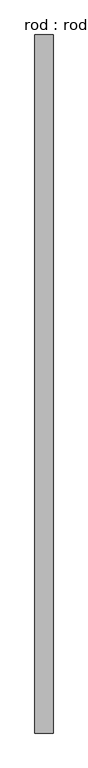
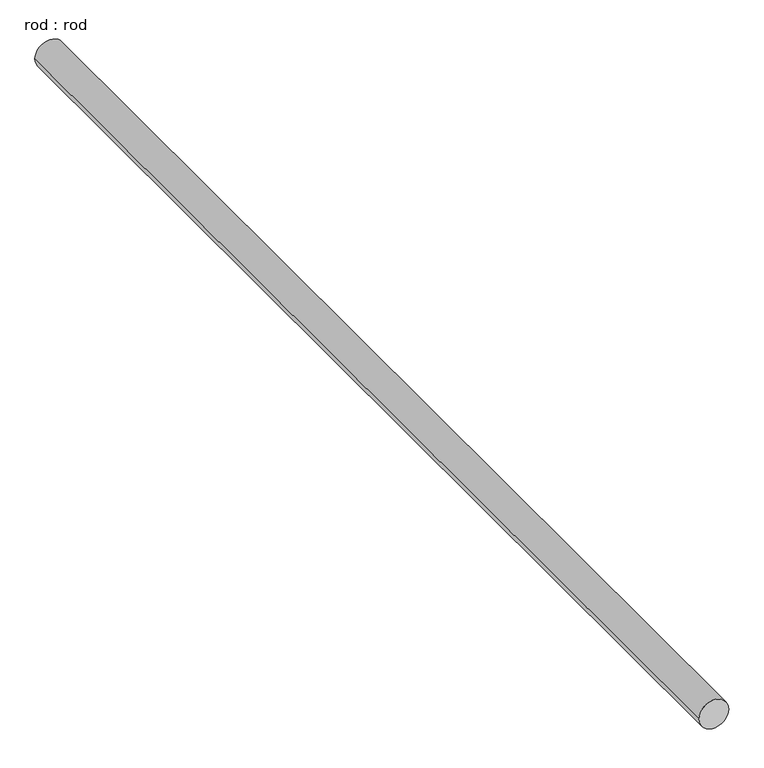
"""IFC4 building model written with IfcOpenShell, lengths in millimetres: proxy geometry, rod : rod."""

from ifc_helpers import new_model, si_unit, point, frame, frame_2d, origin, place, context, project, spatial, circle_curve, trimmed, segment, composite_curve, outline, extrude, source, transform, mapped, element, save


def rod_rod_69a24432(model_context):
    return source(origin(), model_context, "Body", "SweptSolid", [
        extrude(outline(composite_curve([segment(trimmed(circle_curve(frame_2d((0.0108462, 0.0)), 200.0), [point((0.0108462, 200.0))], [point((0.0108462, -200.0))], False, "CARTESIAN"), True, "CONTINUOUS"), segment(trimmed(circle_curve(frame_2d((0.0108462, 0.0)), 200.0), [point((0.0108462, -200.0))], [point((0.0108462, 200.0))], False, "CARTESIAN"), True, "CONTINUOUS")], self_intersect=False)), frame((0.0, -3607.5856259, 0.0), z_axis=(0.0, 1.0, 0.0), x_axis=(0.0, 0.0, 1.0)), (0.0, 0.0, 1.0), 15400.6284824),
    ])


if __name__ == "__main__":
    model = new_model("IFC4")
    model_context = context("Model", 3, world=origin())
    ifc_project = project(units=[si_unit("LENGTHUNIT", "METRE", prefix="MILLI")], contexts=[model_context])
    site = spatial("IfcSite", under=ifc_project)
    building = spatial("IfcBuilding", under=site)
    placement = place(None, origin())
    rod_rod_shape = rod_rod_69a24432(model_context)
    element("IfcBuildingElementProxy", 1, Name="rod : rod", ObjectType="rod : rod", at=placement, inside=building, context=model_context, shape_type="MappedRepresentation", body=[
        mapped(rod_rod_shape, transform((0.0, 0.0, 0.0), x_axis=(1.0, 0.0, 0.0), y_axis=(0.0, 1.0, 0.0), z_axis=(0.0, 0.0, 1.0))),
    ])
    save(model, "model.ifc")

# Revit data of these elements
# Type "rod : rod"
#   Default Elevation = 0
